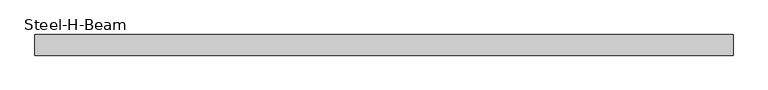
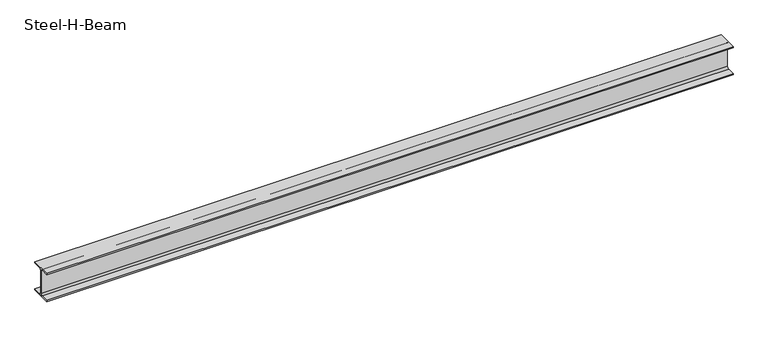
"""IFC4 building model written with IfcOpenShell, lengths in millimetres: beam geometry, Steel-H-Beam : BM121_H-294×200x8x12."""

import ifcopenshell
import ifcopenshell.guid

model = None  # the IFC model being written
_history = None  # IfcOwnerHistory: only IFC2X3 demands one
_inside = {}  # id of a spatial element -> (the spatial element, [elements in it])
_under = {}  # id of a project, library or spatial element -> (it, [spatial elements below it])
_declared = {}  # id of a project -> (the project, [libraries it declares])
_typed = {}  # id of a type object -> (the type object, [elements of that type])
_made_of = {}  # id of a material, layer set ... -> (it, [elements and type objects made of it])


def new_model(schema):
    """Start an empty IFC model of exactly this schema.

    Asked for "IFC4X3", IfcOpenShell would pick the latest addendum, in which some entities
    have other attributes; the version numbers below select the first issue.
    IFC2X3 requires an IfcOwnerHistory on every rooted entity: one is made here for all.
    """
    global model, _history
    if schema == "IFC4X3":
        model = ifcopenshell.file(schema_version=(4, 3, 0, 0))
    else:
        model = ifcopenshell.file(schema=schema)
    _inside.clear()
    _under.clear()
    _declared.clear()
    _typed.clear()
    _made_of.clear()
    _history = None
    if model.schema == "IFC2X3":
        org = make("IfcOrganization", Name="unknown")
        user = make(
            "IfcPersonAndOrganization",
            ThePerson=make("IfcPerson", FamilyName="unknown"),
            TheOrganization=org,
        )
        app = make(
            "IfcApplication",
            ApplicationDeveloper=org,
            Version="unknown",
            ApplicationFullName="unknown",
            ApplicationIdentifier="unknown",
        )
        _history = make(
            "IfcOwnerHistory",
            OwningUser=user,
            OwningApplication=app,
            ChangeAction="ADDED",
            CreationDate=0,
        )
    return model


def make(cls, **values):
    """One entity of the class cls with the attributes given. An attribute that is None is left unset."""
    return model.create_entity(
        cls, **{name: value for name, value in values.items() if value is not None}
    )


def rooted(cls, **values):
    """An entity with a GlobalId (a new one), such as an element, a storey or a relation."""
    return make(cls, GlobalId=ifcopenshell.guid.new(), OwnerHistory=_history, **values)


def si_unit(unit_type, name, prefix=None):
    """IfcSIUnit, for example si_unit("LENGTHUNIT", "METRE", prefix="MILLI")."""
    return make("IfcSIUnit", UnitType=unit_type, Prefix=prefix, Name=name)


def assignment(units):
    """IfcUnitAssignment: the units of a project."""
    return None if units is None else make("IfcUnitAssignment", Units=units)


def point(xyz):
    """IfcCartesianPoint."""
    return None if xyz is None else make("IfcCartesianPoint", Coordinates=xyz)


def direction(xyz):
    """IfcDirection."""
    return None if xyz is None else make("IfcDirection", DirectionRatios=xyz)


def frame(location, z_axis=None, x_axis=None):
    """IfcAxis2Placement3D, a coordinate frame: its origin and axes. An axis left out is left unset."""
    return make(
        "IfcAxis2Placement3D",
        Location=point(location),
        Axis=direction(z_axis),
        RefDirection=direction(x_axis),
    )


def frame_2d(location, x_axis=None):
    """IfcAxis2Placement2D, a coordinate frame in the plane: its origin and x axis."""
    return make(
        "IfcAxis2Placement2D", Location=point(location), RefDirection=direction(x_axis)
    )


def origin():
    """The frame at (0, 0, 0) with its axes left unset."""
    return frame((0.0, 0.0, 0.0))


def place(relative_to, where):
    """IfcLocalPlacement: puts the frame where relative to a parent placement (None: the world)."""
    return make(
        "IfcLocalPlacement", PlacementRelTo=relative_to, RelativePlacement=where
    )


def context(
    kind, dimensions, precision=None, world=None, true_north=None, identifier=None
):
    """IfcGeometricRepresentationContext, for example the 3D "Model" context."""
    return make(
        "IfcGeometricRepresentationContext",
        ContextIdentifier=identifier,
        ContextType=kind,
        CoordinateSpaceDimension=dimensions,
        Precision=precision,
        WorldCoordinateSystem=world,
        TrueNorth=true_north,
    )


def project(units=None, contexts=None):
    """IfcProject with its units and contexts."""
    return rooted(
        "IfcProject",
        Name="project",
        RepresentationContexts=contexts,
        UnitsInContext=assignment(units),
    )


def spatial(cls, under=None, at=None, **own):
    """A site, building, storey or space (cls), placed at a placement, below another one or the project."""
    s = rooted(cls, ObjectPlacement=at, **own)
    if under is not None:
        _under.setdefault(under.id(), (under, []))[1].append(s)
    return s


def polyline(points):
    """IfcPolyline through the points."""
    return make("IfcPolyline", Points=[point(p) for p in points])


def circle_curve(where, radius):
    """IfcCircle in the frame where."""
    return make("IfcCircle", Position=where, Radius=radius)


def trimmed(basis, trim1, trim2, sense, master):
    """IfcTrimmedCurve: the piece of a basis curve between two trims."""
    return make(
        "IfcTrimmedCurve",
        BasisCurve=basis,
        Trim1=trim1,
        Trim2=trim2,
        SenseAgreement=sense,
        MasterRepresentation=master,
    )


def segment(curve, same_sense, transition):
    """IfcCompositeCurveSegment."""
    return make(
        "IfcCompositeCurveSegment",
        Transition=transition,
        SameSense=same_sense,
        ParentCurve=curve,
    )


def composite_curve(segments, self_intersect=None):
    """IfcCompositeCurve: segments joined end to end."""
    return make("IfcCompositeCurve", Segments=segments, SelfIntersect=self_intersect)


def outline(outer, holes=None, kind="AREA"):
    """IfcArbitraryClosedProfileDef: a profile drawn as a closed curve; with holes, ...WithVoids."""
    if holes is None:
        return make("IfcArbitraryClosedProfileDef", ProfileType=kind, OuterCurve=outer)
    return make(
        "IfcArbitraryProfileDefWithVoids",
        ProfileType=kind,
        OuterCurve=outer,
        InnerCurves=holes,
    )


def extrude(swept, where, along, depth):
    """IfcExtrudedAreaSolid: the profile swept, set in the frame where, extruded along a direction by depth."""
    return make(
        "IfcExtrudedAreaSolid",
        SweptArea=swept,
        Position=where,
        ExtrudedDirection=direction(along),
        Depth=depth,
    )


def shape(context_of_items, identifier, shape_type, items):
    """IfcShapeRepresentation: the items that make up one representation, for example the "Body"."""
    return make(
        "IfcShapeRepresentation",
        ContextOfItems=context_of_items,
        RepresentationIdentifier=identifier,
        RepresentationType=shape_type,
        Items=items,
    )


def source(mapping_origin, context_of_items, identifier, shape_type, items):
    """IfcRepresentationMap: a shape defined once, which mapped items show again and again."""
    return make(
        "IfcRepresentationMap",
        MappingOrigin=mapping_origin,
        MappedRepresentation=shape(context_of_items, identifier, shape_type, items),
    )


def transform(
    local_origin,
    x_axis=None,
    y_axis=None,
    z_axis=None,
    scale=None,
    scale2=None,
    scale3=None,
    uniform=True,
):
    """IfcCartesianTransformationOperator3D, or its non-uniform kind. x_axis, y_axis, z_axis: its Axis1, 2, 3."""
    if uniform:
        return make(
            "IfcCartesianTransformationOperator3D",
            Axis1=direction(x_axis),
            Axis2=direction(y_axis),
            LocalOrigin=point(local_origin),
            Scale=scale,
            Axis3=direction(z_axis),
        )
    return make(
        "IfcCartesianTransformationOperator3DnonUniform",
        Axis1=direction(x_axis),
        Axis2=direction(y_axis),
        LocalOrigin=point(local_origin),
        Scale=scale,
        Axis3=direction(z_axis),
        Scale2=scale2,
        Scale3=scale3,
    )


def mapped(mapping_source, mapping_target):
    """IfcMappedItem: shows the shape of a source again, moved by a transform."""
    return make(
        "IfcMappedItem", MappingSource=mapping_source, MappingTarget=mapping_target
    )


def made_of(thing, what):
    """Note that an element or type object is made of a material, layer set ...; save() writes the relation."""
    if what is not None:
        _made_of.setdefault(what.id(), (what, []))[1].append(thing)
    return thing


def element(
    cls,
    number,
    at=None,
    inside=None,
    cuts=None,
    type_object=None,
    material=None,
    context=None,
    identifier="Body",
    shape_type=None,
    held_by="IfcProductDefinitionShape",
    body=None,
    shapes=None,
    **own,
):
    """One element of the class cls, such as IfcWall. Its Tag is "e" and its number.

    at: its placement. inside: the storey or other place that contains it. cuts: it is an
    opening in that element (IfcRelVoidsElement). A single representation is given by context,
    identifier, shape_type and body (its items); several are given by shapes. held_by: the class
    of the entity that holds the representations. save() writes the other relations.
    """
    e = rooted(cls, Tag="e%d" % number, ObjectPlacement=at, **own)
    if body is not None:
        shapes = [shape(context, identifier, shape_type, body)]
    if shapes is not None:
        e.Representation = make(held_by, Representations=shapes)
    if inside is not None:
        _inside.setdefault(inside.id(), (inside, []))[1].append(e)
    if cuts is not None:
        rooted(
            "IfcRelVoidsElement", RelatingBuildingElement=cuts, RelatedOpeningElement=e
        )
    if type_object is not None:
        _typed.setdefault(type_object.id(), (type_object, []))[1].append(e)
    return made_of(e, material)


def aggregate(whole, parts):
    """IfcRelAggregates: a whole, such as a stair, and the parts it consists of."""
    return rooted("IfcRelAggregates", RelatingObject=whole, RelatedObjects=parts)


def save(model, path):
    """Write the relations noted so far, then the file.

    IfcRelAggregates (storeys below a building ...), IfcRelContainedInSpatialStructure (elements
    in a storey), IfcRelDefinesByType, IfcRelAssociatesMaterial and IfcRelDeclares: one each for
    every whole, place, type object, material and project.
    """
    for whole, parts in _under.values():
        aggregate(whole, parts)
    for where, things in _inside.values():
        rooted(
            "IfcRelContainedInSpatialStructure",
            RelatedElements=things,
            RelatingStructure=where,
        )
    for kind, things in _typed.values():
        rooted("IfcRelDefinesByType", RelatedObjects=things, RelatingType=kind)
    for what, things in _made_of.values():
        rooted("IfcRelAssociatesMaterial", RelatedObjects=things, RelatingMaterial=what)
    for by, libraries in _declared.values():
        rooted("IfcRelDeclares", RelatingContext=by, RelatedDefinitions=libraries)
    model.write(path)


def steel_h_beam_013c60b8(model_context):
    return source(origin(), model_context, "Body", "SweptSolid", [
        extrude(outline(composite_curve([segment(polyline([(100.0, -135.0), (100.0, -147.0), (-100.0, -147.0), (-100.0, -135.0), (-22.0, -135.0)]), True, "CONTINUOUS"), segment(trimmed(circle_curve(frame_2d((-22.0, -117.0)), 18.0), [point((-22.0, -135.0))], [point((-4.0, -117.0))], True, "CARTESIAN"), True, "CONTINUOUS"), segment(polyline([(-4.0, -117.0), (-4.0, 117.0)]), True, "CONTINUOUS"), segment(trimmed(circle_curve(frame_2d((-22.0, 117.0)), 18.0), [point((-4.0, 117.0))], [point((-22.0, 135.0))], True, "CARTESIAN"), True, "CONTINUOUS"), segment(polyline([(-22.0, 135.0), (-100.0, 135.0), (-100.0, 147.0), (100.0, 147.0), (100.0, 135.0), (22.0, 135.0)]), True, "CONTINUOUS"), segment(trimmed(circle_curve(frame_2d((22.0, 117.0)), 18.0), [point((22.0, 135.0))], [point((4.0, 117.0))], True, "CARTESIAN"), True, "CONTINUOUS"), segment(polyline([(4.0, 117.0), (4.0, -117.0)]), True, "CONTINUOUS"), segment(trimmed(circle_curve(frame_2d((22.0, -117.0)), 18.0), [point((4.0, -117.0))], [point((22.0, -135.0))], True, "CARTESIAN"), True, "CONTINUOUS"), segment(polyline([(22.0, -135.0), (100.0, -135.0)]), True, "CONTINUOUS")], self_intersect=False)), frame((-3380.0, 0.0, 0.0), z_axis=(1.0, 0.0, 0.0), x_axis=(0.0, 1.0, 0.0)), (0.0, 0.0, 1.0), 6760.0),
    ])


if __name__ == "__main__":
    model = new_model("IFC4")
    model_context = context("Model", 3, world=origin())
    ifc_project = project(units=[si_unit("LENGTHUNIT", "METRE", prefix="MILLI")], contexts=[model_context])
    site = spatial("IfcSite", under=ifc_project)
    building = spatial("IfcBuilding", under=site)
    placement = place(None, origin())
    steel_h_beam_shape = steel_h_beam_013c60b8(model_context)
    element("IfcBeam", 1, ObjectType="Steel-H-Beam : BM121_H-294×200x8x12", at=placement, inside=building, context=model_context, shape_type="MappedRepresentation", body=[
        mapped(steel_h_beam_shape, transform((0.0, 0.0, 0.0), x_axis=(1.0, 0.0, 0.0), y_axis=(0.0, 1.0, 0.0), z_axis=(0.0, 0.0, 1.0))),
    ])
    save(model, "model.ifc")

# Revit data of these elements
# Project information
#   Project ISM Data = "<?xml version=\"1.0\" encoding=\"utf-16\"?><ism schema_version=\"03.00\"><section_positioning><element family_name=\"CO_RC_REC\" symbol_name=\"CCC12_Rec_450x450\" section_id=\"F2ADF140-E21A-4820-8170-6F63D956DCAD\" category=\"OST_StructuralColumns\" mirror_y=\"0\" mirror_x=\"0\" /><element family_name=\"CO_RC_REC\" symbol_name=\"CCC12_Rec_450x450\" section_id=\"B35A310E-4F33-462b-819C-3ADD300C0CEB\" category=\"OST_StructuralColumns\" mirror_y=\"0\" mirror_x=\"0\" /><element family_name=\"CO_RC_REC\" symbol_name=\"CCC12_Rec_450x450\" section_id=\"711054EC-0DB2-46e3-AD20-004560300C00\" category=\"OST_StructuralColumns\" mirror_y=\"0\" mirror_x=\"0\" /><element family_name=\"CO_RC_REC\" symbol_name=\"300 x 450\" section_id=\"B5C54EC9-8EBD-4860-AB72-EF5791AED394\" category=\"OST_StructuralColumns\" mirror_y=\"0\" mirror_x=\"0\" /><element family_name=\"GI_RC_C\" symbol_name=\"SGC11_400x500\" section_id=\"0A7B8D02-9EA4-4aa9-A41A-E30BB5B6B6C5\" category=\"OST_StructuralFraming\" mirror_y=\"0\" mirror_x=\"0\" /><element family_name=\"GI_RC_C\" symbol_name=\"SGC11_400x500\" section_id=\"714BBD27-DB58-47da-B54C-5806291C2D3C\" category=\"OST_StructuralFraming\" mirror_y=\"0\" mirror_x=\"0\" /><element family_name=\"GI_RC_C\" symbol_name=\"SGC11_400x500\" section_id=\"F36E62C1-13EE-4807-A3C1-899E23E0BEDE\" category=\"OST_StructuralFraming\" mirror_y=\"0\" mirror_x=\"0\" /><element family_name=\"GI_RC_C\" symbol_name=\"SGC11_400x500\" section_id=\"F5448801-679E-44d6-8F46-E676344F8165\" category=\"OST_StructuralFraming\" mirror_y=\"0\" mirror_x=\"0\" /><element family_name=\"GI_RC_C\" symbol_name=\"SGC11_400x600\" section_id=\"05D74241-6318-4cac-95F5-7B878260D5B5\" category=\"OST_StructuralFraming\" mirror_y=\"0\" mirror_x=\"0\" /><element family_name=\"GI_RC_C\" symbol_name=\"SGC11_400x500\" section_id=\"846DCB0C-E06B-4978-9D43-E1CC0FDE7595\" category=\"OST_StructuralFraming\" mirror_y=\"0\" mirror_x=\"0\" /><element family_name=\"GI_RC_C\" symbol_name=\"SGC11_400x500\" section_id=\"2ADF82B8-986D-4f44-85DE-89D921292160\" category=\"OST_StructuralFraming\" mirror_y=\"0\" mirror_x=\"0\" /><element family_name=\"GI_RC_C\" symbol_name=\"SGC11_400x500\" section_id=\"7AF371ED-051B-4a30-8826-11F11C212B73\" category=\"OST_StructuralFraming\" mirror_y=\"0\" mirror_x=\"0\" /><element family_name=\"GI_RC_C\" symbol_name=\"SGC11_400x500\" section_id=\"2FE74006-ADDA-412f-A522-853919E62B4D\" category=\"OST_StructuralFraming\" mirror_y=\"0\" mirror_x=\"0\" /><element family_name=\"GI_RC_C\" symbol_name=\"SGC11_400x500\" section_id=\"09B63641-D581-4a6c-A18E-54C17EC989A4\" category=\"OST_StructuralFraming\" mirror_y=\"0\" mirror_x=\"0\" /><element family_name=\"GI_RC_C\" symbol_name=\"SGC11_400x500\" section_id=\"0DD6B52A-77D0-45a1-82B1-8236ED57078C\" category=\"OST_StructuralFraming\" mirror_y=\"0\" mirror_x=\"0\" /><element family_name=\"GI_RC_C\" symbol_name=\"SGC11_400x500\" section_id=\"35D311D2-DEB8-4469-97DE-110B6DF5B84D\" category=\"OST_StructuralFraming\" mirror_y=\"0\" mirror_x=\"0\" /><element family_name=\"GI_RC_C\" symbol_name=\"SGC11_400x500\" section_id=\"0D3CCDE5-CFF9-431b-A4BD-01BF6636D6BD\" category=\"OST_StructuralFraming\" mirror_y=\"0\" mirror_x=\"0\" /><element family_name=\"GI_RC_C\" symbol_name=\"SGC11_400x500\" section_id=\"C62B2A5B-024A-47ac-B030-C17A67E64A7B\" category=\"OST_StructuralFraming\" mirror_y=\"0\" mirror_x=\"0\" /><element family_name=\"GI_RC_C\" symbol_name=\"SGC11_400x500\" section_id=\"944C6E43-E607-48c3-8358-9E6CB88346E7\" category=\"OST_StructuralFraming\" mirror_y=\"0\" mirror_x=\"0\" /><element family_name=\"GI_RC_C\" symbol_name=\"SGC11_400x500\" section_id=\"A4B1F42D-B1C2-4ad2-8AD6-DB0D5E05998D\" category=\"OST_StructuralFraming\" mirror_y=\"0\" mirror_x=\"0\" /><element family_name=\"GI_RC_C\" symbol_name=\"SGC11_400x500\" section_id=\"007E6C70-1139-4b48-B003-C76FAD4C249A\" category=\"OST_StructuralFraming\" mirror_y=\"0\" mirror_x=\"0\" /><element family_name=\"GI_RC_C\" symbol_name=\"SGC11_400x500\" section_id=\"9941AC94-F03A-464c-9912-04590E0C31E0\" category=\"OST_StructuralFraming\" mirror_y=\"0\" mirror_x=\"0\" /><element family_name=\"GI_RC_C\" symbol_name=\"SGC11_400x500\" section_id=\"CFD98B8D-8FF4-4e71-A909-0FE7DBCE924E\" category=\"OST_StructuralFraming\" mirror_y=\"0\" mirror_x=\"0\" /><element family_name=\"GI_RC_C\" symbol_name=\"SGC11_400x500\" section_id=\"58262161-98E6-45c8-B2BD-4508105FF662\" category=\"OST_StructuralFraming\" mirror_y=\"0\" mirror_x=\"0\" /><element family_name=\"GI_RC_C\" symbol_name=\"SGC11_400x500\" section_id=\"66AB4841-610A-4883-97F7-1282A56484E1\" category=\"OST_StructuralFraming\" mirror_y=\"0\" mirror_x=\"0\" /><element family_name=\"GI_RC_C\" symbol_name=\"SGC11_400x500\" section_id=\"D2B324BE-BBD6-49da-9730-60EA7AD4D3A0\" category=\"OST_StructuralFraming\" mirror_y=\"0\" mirror_x=\"0\" /><element family_name=\"GI_RC_C\" symbol_name=\"SGC11_400x500\" section_id=\"92A8ECE7-C053-46b1-92ED-F2C041617E7B\" category=\"OST_StructuralFraming\" mirror_y=\"0\" mirror_x=\"0\" /><element family_name=\"GI_RC_C\" symbol_name=\"SGC11_400x500\" section_id=\"B4C4BDB0-65C4-4016-9C78-DBD77E229523\" category=\"OST_StructuralFraming\" mirror_y=\"0\" mirror_x=\"0\" /><element family_name=\"GI_RC_C\" symbol_name=\"SGC11_400x500\" section_id=\"57270646-162F-4c83-BDB7-A5FBEA9120BD\" category=\"OST_StructuralFraming\" mirror_y=\"0\" mirror_x=\"0\" /><element family_name=\"GI_RC_C\" symbol_name=\"SGC11_400x500\" section_id=\"BDEF733F-00AA-4eee-B6C6-50229FC1D236\" category=\"OST_StructuralFraming\" mirror_y=\"0\" mirror_x=\"0\" /><element family_name=\"GI_RC_C\" symbol_name=\"SGC11_400x500\" section_id=\"84A94E1E-3074-40f4-9690-97191755F019\" category=\"OST_StructuralFraming\" mirror_y=\"0\" mirror_x=\"0\" /><element family_name=\"GI_RC_C\" symbol_name=\"SGC11_400x500\" section_id=\"8A7D913D-7967-4718-912D-B83DF0AD2EDD\" category=\"OST_StructuralFraming\" mirror_y=\"0\" mirror_x=\"0\" /><element family_name=\"GI_RC_C\" symbol_name=\"SGC11_400x500\" section_id=\"83553D70-90FA-469c-B5C3-EF03F3FC6475\" category=\"OST_StructuralFraming\" mirror_y=\"0\" mirror_x=\"0\" /><element family_name=\"GI_RC_C\" symbol_name=\"SGC11_400x500\" section_id=\"6880C1E4-C50B-4c1b-B61C-23F2D8C46873\" category=\"OST_StructuralFraming\" mirror_y=\"0\" mirror_x=\"0\" /><element family_name=\"GI_RC_C\" symbol_name=\"SGC11_400x500\" section_id=\"08594C43-CD40-47de-A3BA-8BFB47F64994\" category=\"OST_StructuralFraming\" mirror_y=\"0\" mirror_x=\"0\" /><element family_name=\"GI_RC_C\" symbol_name=\"SGC11_400x500\" section_id=\"7D2E11FA-A5E1-4434-B9BE-AABA1A16CA03\" category=\"OST_StructuralFraming\" mirror_y=\"0\" mirror_x=\"0\" /><element family_name=\"GI_RC_C\" symbol_name=\"SGC11_400x500\" section_id=\"D892DFA4-5441-4ad2-A390-253492293B1B\" category=\"OST_StructuralFraming\" mirror_y=\"0\" mirror_x=\"0\" /><element family_name=\"GI_RC_C\" symbol_name=\"SGC11_400x500\" section_id=\"E5A32FE6-89C4-49f1-B3B9-1CABE7C48A4D\" category=\"OST_StructuralFraming\" mirror_y=\"0\" mirror_x=\"0\" /><element family_name=\"GI_RC_C\" symbol_name=\"SGC11_400x500\" section_id=\"8AE872C2-5DBE-47c5-934B-7E964A84B589\" category=\"OST_StructuralFraming\" mirror_y=\"0\" mirror_x=\"0\" /><element family_name=\"GI_RC_C\" symbol_name=\"SGC11_400x500\" section_id=\"3C847B60-488A-4604-A400-16A3A65E919B\" category=\"OST_StructuralFraming\" mirror_y=\"0\" mirror_x=\"0\" /><element family_name=\"GI_RC_C\" symbol_name=\"SGC11_400x500\" section_id=\"DBEC432A-3F7B-4266-AD99-2A937DC70BCF\" category=\"OST_StructuralFraming\" mirror_y=\"0\" mirror_x=\"0\" /><element family_name=\"GI_RC_C\" symbol_name=\"SGC11_400x500\" section_id=\"59403DD6-7A51-48aa-A3BE-962457E6F10E\" category=\"OST_StructuralFraming\" mirror_y=\"0\" mirror_x=\"0\" /><element family_name=\"GI_RC_C\" symbol_name=\"SGC11_400x500\" section_id=\"11CDDF5D-38B6-43b2-A291-FC188BE232BC\" category=\"OST_StructuralFraming\" mirror_y=\"0\" mirror_x=\"0\" /><element family_name=\"GI_RC_C\" symbol_name=\"SGC11_400x500\" section_id=\"10BF2843-EFC9-4136-933C-5B270D970277\" category=\"OST_StructuralFraming\" mirror_y=\"0\" mirror_x=\"0\" /><element family_name=\"GI_RC_C\" symbol_name=\"SGC11_400x500\" section_id=\"E1B09A9C-F6C6-47d9-976B-E313C0E3F52B\" category=\"OST_StructuralFraming\" mirror_y=\"0\" mirror_x=\"0\" /><element family_name=\"GI_RC_C\" symbol_name=\"SGC11_400x500\" section_id=\"A3A22EC3-26C8-4588-A0AB-AFAE02DF267E\" category=\"OST_StructuralFraming\" mirror_y=\"0\" mirror_x=\"0\" /><element family_name=\"GI_RC_C\" symbol_name=\"SGC11_400x500\" section_id=\"114828FC-BDC1-4343-9119-BCB5395DAA64\" category=\"OST_StructuralFraming\" mirror_y=\"0\" mirror_x=\"0\" /><element family_name=\"GI_RC_C\" symbol_name=\"SGC11_400x500\" section_id=\"797626F9-3558-4623-826F-15FB93088CB3\" category=\"OST_StructuralFraming\" mirror_y=\"0\" mirror_x=\"0\" /><element family_name=\"GI_RC_C\" symbol_name=\"SGC11_400x500\" section_id=\"4BF369CD-DF09-4346-96CB-C6C6380A2599\" category=\"OST_StructuralFraming\" mirror_y=\"0\" mirror_x=\"0\" /><element family_name=\"GI_RC_C\" symbol_name=\"SGC11_400x500\" section_id=\"722B46BA-61C4-44a1-9ECF-325B60B6688D\" category=\"OST_StructuralFraming\" mirror_y=\"0\" mirror_x=\"0\" /><element family_name=\"GI_RC_C\" symbol_name=\"SGC11_400x500\" section_id=\"C33DBE84-19C1-4379-AB6E-A41F7420F18C\" category=\"OST_StructuralFraming\" mirror_y=\"0\" mirror_x=\"0\" /><element family_name=\"GI_RC_C\" symbol_name=\"SGC11_400x500\" section_id=\"1F2D3B75-66F2-4d88-A1DD-647969477B86\" category=\"OST_StructuralFraming\" mirror_y=\"0\" mirror_x=\"0\" /><element family_name=\"GI_RC_C\" symbol_name=\"SGC11_400x500\" section_id=\"DFBF96B2-410A-4f39-80C4-D8CF78561C93\" category=\"OST_StructuralFraming\" mirror_y=\"0\" mirror_x=\"0\" /><element family_name=\"GI_RC_C\" symbol_name=\"SGC11_400x500\" section_id=\"D6793CD3-AB64-417c-9C28-8B18A0A2D336\" category=\"OST_StructuralFraming\" mirror_y=\"0\" mirror_x=\"0\" /><element family_name=\"GI_RC_C\" symbol_name=\"SGC11_400x500\" section_id=\"90884AC0-EA00-4caa-86E1-E6B886FD90ED\" category=\"OST_StructuralFraming\" mirror_y=\"0\" mirror_x=\"0\" /><element family_name=\"GI_RC_C\" symbol_name=\"SGC11_400x500\" section_id=\"64BC7B89-F7C8-4dae-A5C8-F10DF9E5F6BA\" category=\"OST_StructuralFraming\" mirror_y=\"0\" mirror_x=\"0\" /><element family_name=\"GI_RC_C\" symbol_name=\"SGC11_400x500\" section_id=\"D82E4D85-2728-40e5-9F60-1C7FB2990D78\" category=\"OST_StructuralFraming\" mirror_y=\"0\" mirror_x=\"0\" /><element family_name=\"GI_RC_C\" symbol_name=\"SGC11_400x500\" section_id=\"1E6D05B9-BF84-4669-AA27-948ADA1D511E\" category=\"OST_StructuralFraming\" mirror_y=\"0\" mirror_x=\"0\" /><element family_name=\"GI_RC_C\" symbol_name=\"SGC11_400x500\" section_id=\"73608CB2-EB94-466e-883D-814030EF49D6\" category=\"OST_StructuralFraming\" mirror_y=\"0\" mirror_x=\"0\" /><element family_name=\"GI_RC_C\" symbol_name=\"SGC11_400x500\" section_id=\"4EAF07EF-4E08-4065-9F08-BF69D4413867\" category=\"OST_StructuralFraming\" mirror_y=\"1\" mirror_x=\"1\" /></section_positioning><surface_member_mappings /><element_binding><element revit_id=\"0aa8b22b-49cd-4eb2-b994-d423f7aad482-0014435e\" ism_id=\"637A3C89-B4B9-4EE4-9E04-FF73E7A5771D\" /><element revit_id=\"af7cfdda-f71a-4a09-bb03-63e0c16d5d93-00152efa\" ism_id=\"088C1743-AFAE-4D55-B14F-2330F3A79060\" /><element revit_id=\"af7cfdda-f71a-4a09-bb03-63e0c16d5d93-00152efc\" ism_id=\"38278b30-864a-4bde-bfee-6c2d4309b281\" /><element revit_id=\"af7cfdda-f71a-4a09-bb03-63e0c16d5d93-00152eff\" ism_id=\"e2895b00-887b-4cf1-92a9-c4855f67b579\" /><element revit_id=\"af7cfdda-f71a-4a09-bb03-63e0c16d5d93-00152f02\" ism_id=\"a6b13b86-1938-47ee-8937-754844bb71d9\" /><element revit_id=\"af7cfdda-f71a-4a09-bb03-63e0c16d5d93-00152f05\" ism_id=\"b3cdb4ae-01be-49a8-8521-dfb37fcb7a09\" /><element revit_id=\"af7cfdda-f71a-4a09-bb03-63e0c16d5d93-00152f08\" ism_id=\"0a200294-2d0f-43b2-a10b-c345be42008c\" /><element revit_id=\"af7cfdda-f71a-4a09-bb03-63e0c16d5d
#     93-00152f0a\" ism_id=\"434ac00d-0b75-408a-b526-bf8655b26baf\" /><element revit_id=\"af7cfdda-f71a-4a09-bb03-63e0c16d5d93-00152f0c\" ism_id=\"5e4f7e2a-2154-47cc-93bc-24e7bd197632\" /><element revit_id=\"af7cfdda-f71a-4a09-bb03-63e0c16d5d93-00152f0e\" ism_id=\"f1998cd9-044c-4f7a-99e6-248bc5b45dba\" /><element revit_id=\"af7cfdda-f71a-4a09-bb03-63e0c16d5d93-00152f10\" ism_id=\"6ca0e144-6dd7-4824-b6a4-c3599ffcc64c\" /><element revit_id=\"af7cfdda-f71a-4a09-bb03-63e0c16d5d93-00152f12\" ism_id=\"173f1f07-ca52-4750-b7f6-1ef0180c36ba\" /><element revit_id=\"af7cfdda-f71a-4a09-bb03-63e0c16d5d93-00152f15\" ism_id=\"29a619d1-86ac-46c7-a220-2e78769b313e\" /><element revit_id=\"af7cfdda-f71a-4a09-bb03-63e0c16d5d93-00152f17\" ism_id=\"de21b25d-6b5e-4da6-89ee-8b671f1287ec\" /><element revit_id=\"af7cfdda-f71a-4a09-bb03-63e0c16d5d93-00152f19\" ism_id=\"70cdf538-eeaa-48c4-9315-181e56578638\" /><element revit_id=\"af7cfdda-f71a-4a09-bb03-63e0c16d5d93-00152f1b\" ism_id=\"49734cf8-a963-4163-b104-a25bff74fff0\" /><element revit_id=\"af7cfdda-f71a-4a09-bb03-63e0c16d5d93-00152f1d\" ism_id=\"a5a98e28-e98d-4759-bcab-d40632bfc19f\" /><element revit_id=\"af7cfdda-f71a-4a09-bb03-63e0c16d5d93-00152f1f\" ism_id=\"ab6af08f-90da-4d2f-a66a-db65621b8e94\" /><element revit_id=\"af7cfdda-f71a-4a09-bb03-63e0c16d5d93-00152f21\" ism_id=\"a65b64ab-134d-4223-82b7-5e66d90bc276\" /><element revit_id=\"af7cfdda-f71a-4a09-bb03-63e0c16d5d93-00152f23\" ism_id=\"6a1f317f-8940-4af8-9522-8e6c47c0c3a6\" /><element revit_id=\"af7cfdda-f71a-4a09-bb03-63e0c16d5d93-00152f25\" ism_id=\"880c6aab-7058-4382-9d83-6c759bdcf822\" /><element revit_id=\"af7cfdda-f71a-4a09-bb03-63e0c16d5d93-00152f27\" ism_id=\"555977b1-6494-4ee8-b235-8bae97762787\" /><element revit_id=\"af7cfdda-f71a-4a09-bb03-63e0c16d5d93-00152f29\" ism_id=\"66c9b467-8c65-4f1e-9542-95b43d793e9b\" /><element revit_id=\"af7cfdda-f71a-4a09-bb03-63e0c16d5d93-00152f2b\" ism_id=\"217a9ce2-64ab-4115-836e-06014fa1b21e\" /><element revit_id=\"af7cfdda-f71a-4a09-bb03-63e0c16d5d93-00152f2d\" ism_id=\"f7fc30da-832d-44e7-bab3-dd115d25639e\" /><element revit_id=\"af7cfdda-f71a-4a09-bb03-63e0c16d5d93-00152f2f\" ism_id=\"715eb46c-1b8d-4226-a7c6-6c6c165bf34d\" /><element revit_id=\"af7cfdda-f71a-4a09-bb03-63e0c16d5d93-00152f31\" ism_id=\"ef53c2b2-6fcf-42d2-96ea-f30a899bf64f\" /><element revit_id=\"af7cfdda-f71a-4a09-bb03-63e0c16d5d93-00152f34\" ism_id=\"1aefa093-18ee-4a97-8178-1b1fb4b7aceb\" /><element revit_id=\"af7cfdda-f71a-4a09-bb03-63e0c16d5d93-00152f38\" ism_id=\"262f02a9-64ca-487b-befd-4b58d44dffa7\" /><element revit_id=\"af7cfdda-f71a-4a09-bb03-63e0c16d5d93-00152f3b\" ism_id=\"6f2442a8-c4c0-4b53-9d7f-7059d6ededd2\" /><element revit_id=\"af7cfdda-f71a-4a09-bb03-63e0c16d5d93-00152f3e\" ism_id=\"dd838df4-69c7-406c-93e1-418c01f5734f\" /><element revit_id=\"af7cfdda-f71a-4a09-bb03-63e0c16d5d93-00152f40\" ism_id=\"9dec5077-28a7-4c32-95d2-08813de6a916\" /><element revit_id=\"af7cfdda-f71a-4a09-bb03-63e0c16d5d93-00152f42\" ism_id=\"9370ae5f-9277-4bb3-917b-cb3f318800a8\" /><element revit_id=\"af7cfdda-f71a-4a09-bb03-63e0c16d5d93-00152f44\" ism_id=\"0f3f2c81-58b4-4698-b1be-75061a4a2ae1\" /><element revit_id=\"af7cfdda-f71a-4a09-bb03-63e0c16d5d93-00152f46\" ism_id=\"95dca10f-6510-4ae7-a23e-7a1fd6939662\" /><element revit_id=\"af7cfdda-f71a-4a09-bb03-63e0c16d5d93-00152f49\" ism_id=\"83bad907-6a1c-4702-9990-a1a9c13d0160\" /><element revit_id=\"af7cfdda-f71a-4a09-bb03-63e0c16d5d93-00152f4d\" ism_id=\"7dba72dc-0de8-457c-8d3c-9c80941133ff\" /><element revit_id=\"af7cfdda-f71a-4a09-bb03-63e0c16d5d93-00152f51\" ism_id=\"a6cf3de2-949b-45b4-8029-061e06e5ab91\" /><element revit_id=\"af7cfdda-f71a-4a09-bb03-63e0c16d5d93-00152f54\" ism_id=\"77af5754-dd62-4c90-accb-d0b9405b5baf\" /><element revit_id=\"af7cfdda-f71a-4a09-bb03-63e0c16d5d93-00152f56\" ism_id=\"6461cb37-823d-49bb-bea2-3dbd4db85a81\" /><element revit_id=\"af7cfdda-f71a-4a09-bb03-63e0c16d5d93-00152f59\" ism_id=\"e2f2909f-27bc-426e-b2db-27b1217d3560\" /><element revit_id=\"af7cfdda-f71a-4a09-bb03-63e0c16d5d93-00152f5b\" ism_id=\"46c410de-fc65-4593-ae24-da1a154b45fb\" /><element revit_id=\"af7cfdda-f71a-4a09-bb03-63e0c16d5d93-00152f5d\" ism_id=\"d7d73cf7-a31f-421c-bc39-3ba338a334b1\" /><element revit_id=\"af7cfdda-f71a-4a09-bb03-63e0c16d5d93-00152f61\" ism_id=\"6bd81f7b-5fd8-4f19-ad3a-4e009274854c\" /><element revit_id=\"af7cfdda-f71a-4a09-bb03-63e0c16d5d93-00152f64\" ism_id=\"f25b9af0-504f-4aaf-a359-d2bc9d32b683\" /><element revit_id=\"af7cfdda-f71a-4a09-bb03-63e0c16d5d93-00152f66\" ism_id=\"f143dcd3-1cc7-47ae-b4ed-c960a7d1349c\" /><element revit_id=\"af7cfdda-f71a-4a09-bb03-63e0c16d5d93-00152f68\" ism_id=\"296e8d7f-a89b-405a-b793-fc1ea4b11be5\" /><element revit_id=\"af7cfdda-f71a-4a09-bb03-63e0c16d5d93-00152f6b\" ism_id=\"48b24488-3184-439c-b285-73e81edfef17\" /><element revit_id=\"af7cfdda-f71a-4a09-bb03-63e0c16d5d93-00152f6e\" ism_id=\"0db0ccd4-631c-4972-aad8-2fd483c55629\" /><element revit_id=\"af7cfdda-f71a-4a09-bb03-63e0c16d5d93-00152f71\" ism_id=\"ee51bd40-01d8-4a48-92c6-90509a96cad2\" /><element revit_id=\"af7cfdda-f71a-4a09-bb03-63e0c16d5d93-00152f73\" ism_id=\"e5c66ce6-ca9d-4591-9d75-5348307a88bc\" /><element revit_id=\"af7cfdda-f71a-4a09-bb03-63e0c16d5d93-00152f75\" ism_id=\"892d82ae-6f73-4af5-8575-78955f2b6c3b\" /><element revit_id=\"af7cfdda-f71a-4a09-bb03-63e0c16d5d93-00152f78\" ism_id=\"cb5b2a2e-5551-4b87-9d0b-6382c09e6ce2\" /><element revit_id=\"af7cfdda-f71a-4a09-bb03-63e0c16d5d93-00152f7c\" ism_id=\"1177c4ab-d04b-426b-80ba-afa1f1403e20\" /><element revit_id=\"af7cfdda-f71a-4a09-bb03-63e0c16d5d93-00152f7f\" ism_id=\"235d8a18-f10a-44ad-8945-ebb2f02646fa\" /><element revit_id=\"af7cfdda-f71a-4a09-bb03-63e0c16d5d93-00152f83\" ism_id=\"6127db9d-7d4b-44c8-806c-e4f7d278db0c\" /><element revit_id=\"af7cfdda-f71a-4a09-bb03-63e0c16d5d93-00152f86\" ism_id=\"85d79da8-d317-4e5b-88a2-88d20cb73d7d\" /><element revit_id=\"af7cfdda-f71a-4a09-bb03-63e0c16d5d93-00152f89\" ism_id=\"f4105a19-7c5e-4970-9446-50e578b67af2\" /><element revit_id=\"af7cfdda-f71a-4a09-bb03-63e0c16d5d93-00152f8b\" ism_id=\"ab299061-87b1-4edc-8a5c-c55542368f39\" /><element revit_id=\"af7cfdda-f71a-4a09-bb03-63e0c16d5d93-00152f8d\" ism_id=\"43097401-25be-48d4-a7ba-f3c37c1b84e9\" /><element revit_id=\"af7cfdda-f71a-4a09-bb03-63e0c16d5d93-00152f8f\" ism_id=\"fd9214b7-59e9-4736-b544-a37d4c180e24\" /><element revit_id=\"af7cfdda-f71a-4a09-bb03-63e0c16d5d93-00152f91\" ism_id=\"b83d1d95-2d97-4532-8a94-368577601c17\" /><element revit_id=\"af7cfdda-f71a-4a09-bb03-63e0c16d5d93-00152f94\" ism_id=\"9bd5e620-e2eb-4ede-9a8b-b0183e171248\" /><element revit_id=\"af7cfdda-f71a-4a09-bb03-63e0c16d5d93-00152f97\" ism_id=\"d6f9d903-1605-43dc-872c-2f9de6642af6\" /><element revit_id=\"af7cfdda-f71a-4a09-bb03-63e0c16d5d93-00152f99\" ism_id=\"7c236b12-3da8-4ae0-bc99-2aa089118476\" /><element revit_id=\"af7cfdda-f71a-4a09-bb03-63e0c16d5d93-00152f9b\" ism_id=\"2b88d03d-aeef-4f51-b98c-562513d6f6da\" /><element revit_id=\"af7cfdda-f71a-4a09-bb03-63e0c16d5d93-00152f9d\" ism_id=\"6639b07f-6759-4580-bc0a-91cdbc82216d\" /><element revit_id=\"af7cfdda-f71a-4a09-bb03-63e0c16d5d93-00152f9f\" ism_id=\"d17e7cf5-d760-4c38-8bb0-8a57fe45e3ad\" /><element revit_id=\"af7cfdda-f71a-4a09-bb03-63e0c16d5d93-00152fa2\" ism_id=\"6dbdf2a2-22ac-4132-a9ae-8992fe15b0d7\" /><element revit_id=\"af7cfdda-f71a-4a09-bb03-63e0c16d5d93-00152fa4\" ism_id=\"663381be-9f3f-499f-b7c1-64170401ecb3\" /><element revit_id=\"af7cfdda-f71a-4a09-bb03-63e0c16d5d93-00152fa6\" ism_id=\"5ba3ff14-3d24-47a8-9418-aecce16bd943\" /><element revit_id=\"af7cfdda-f71a-4a09-bb03-63e0c16d5d93-00152fa8\" ism_id=\"8f845e6a-1432-4c61-8362-e12c105320fb\" /><element revit_id=\"af7cfdda-f71a-4a09-bb03-63e0c16d5d93-00152faa\" ism_id=\"263897bf-02c2-4ed7-8e3f-2020d545125e\" /><element revit_id=\"af7cfdda-f71a-4a09-bb03-63e0c16d5d93-00152fac\" ism_id=\"f1241312-d990-4c87-92ff-afc1975a3d67\" /><element revit_id=\"af7cfdda-f71a-4a09-bb03-63e0c16d5d93-00152fae\" ism_id=\"5740cb23-0cbc-47ce-acea-31b5a043bf0c\" /><element revit_id=\"af7cfdda-f71a-4a09-bb03-63e0c16d5d93-00152fb0\" ism_id=\"7aeaeafb-f9bc-4bee-b237-caade22069b8\" /><element revit_id=\"af7cfdda-f71a-4a09-bb03-63e0c16d5d93-00152fb3\" ism_id=\"90084dda-e197-4e46-8e5b-4f629a594830\" /><element revit_id=\"af7cfdda-f71a-4a09-bb03-63e0c16d5d93-00152fb5\" ism_id=\"2c392f12-2b50-4bd2-8c41-ef64640e587b\" /><element revit_id=\"af7cfdda-f71a-4a09-bb03-63e0c16d5d93-00152fb7\" ism_id=\"d25284c0-6931-4cbb-8ed3-63397f6a5616\" /><element revit_id=\"af7cfdda-f71a-4a09-bb03-63e0c16d5d93-00152fb9\" ism_id=\"32799d39-e9bc-468c-ac64-a3f2c8e075af\" /><element revit_id=\"af7cfdda-f71a-4a09-bb03-63e0c16d5d93-00152fbb\" ism_id=\"61a092b8-d924-4e61-a1ef-adc051541aaf\" /><element revit_id=\"af7cfdda-f71a-4a09-bb03-63e0c16d5d93-00152fbe\" ism_id=\"ae89ad42-0006-42ee-9328-01a896002b7a\" /><element revit_id=\"af7cfdda-f71a-4a09-bb03-63e0c16d5d93-00152fc0\" ism_id=\"7b4d47fd-5fcd-4692-9b39-36bb95372647\" /><element revit_id=\"af7cfdda-f71a-4a09-bb03-63e0c16d5d93-00152fc2\" ism_id=\"150f022d-eb78-47d8-8d70-c7ea5433f366\" /><element revit_id=\"af7cfdda-f71a-4a09-bb03-63e0c16d5d93-00152fc4\" ism_id=\"6780451e-52c6-4962-8bb4-f1fd57bf7865\" /><element revit_id=\"af7cfdda-f71a-4a09-bb03-63e0c16d5d93-00152fc6\" ism_id=\"b3896748-2d7c-424b-ae81-8b769d840fbc\" /><element revit_id=\"af7cfdda-f71a-4a09-bb03-63e0c16d5d93-00152fc9\" ism_id=\"0c64c745-ce95-4f37-8a9d-d07fd5d17ecb\" /><element revit_id=\"af7cfdda-f71a-4a09-bb03-63e0c16d5d93-00152fcc\" ism_id=\"dc23390d-d501-4d7e-9369-f7793a7306a7\" /><element revit_id=\"af7cfdda-f71a-4a09-bb03-63e0c16d5d93-00152fcf\" ism_id=\"a2d2dfc7-08e7-459b-9de9-2d46c1b9d65d\" /><element revit_id=\"af7cfdda-f71a-4a09-bb03-63e0c16d5d93-00152fd2\" ism_id=\"0357c393-c221-46b8-a525-7eece05024d5\" /><element revit_id=\"af7cfdda-f71a-4a09-bb03-63e0c16d5d93-00152fd4\" ism_id=\"7514ec1a-cc54-428f-bbfe-53465c7b9971\" /><element revit_id=\"af7cfdda-f71a-4a09-bb03-63e0c16d5d93-00152fd7\" ism_id=\"f5e61f1a-565d-4eed-b8cc-74798bf49f83\" /><element revit_id=\"af7cfdda-f71a-4a09-bb03-63e0c16d5d93-00152fd9\" ism_id=\"7d7031a0-6061-49e6-8bb3-df1503ddb602\" /><element revit_id=\"af7cfdda-f71a-4a09-bb03-63e0c16d5d93-00152fdb\" ism_id=\"0d733cbc-e2dd-44ec-a5f3-da43d2d7ec46\" /><element revit_id=\"af7cfdda-f71a-4a09-bb03-63e0c16d5d93-00152fdd\" ism_id=\"21cbc8e9-c640-4a2e-8958-1d3b7a784879\" /><element revit_id=\"af7cfdda-f71a-4a09-bb03-63e0c16d5d93-00152fdf\" ism_id=\"fac86bbb-1d81-4320-81cd-30997be31eb4\" /><element revit_id=\"af7cfdda-f71a-4a09-bb03-63e0c16d5d93-00152fe1\" ism_id=\"ebc7c696-170e-4ba4-8599-103279d331b8\" /><element revit_id=\"af7cfdda-f71a-4a09-bb03-63e0c16d5d93-00152fe3\" ism_id=\"91dec439-7fd8-4259-bbce-df46237765e2\" /><element revit_id=\"af7cfdda-f71a-4a09-bb03-63e0c16d5d93-00152fe5\" ism_id=\"6227503a-c521-4b5a-b5c3-b9e2ea2b5c81\" /><element revit_id=\"af7cfdda-f71a-4a09-bb03-63e0c16d5d93-00152fe7\" ism_id=\"e6e91966-53ab-4536-84a0-3f6e5a22fbeb\" /><element revit_id=\"af7cfdda-f71a-4a09-bb03-63e0c16d5d93-00152fe9\" ism_id=\"fb3387b3-301c-40a5-8217-97be67c50843\" /><element revit_id=\"af7cfdda-f71a-4a09-bb03-63e0c16d5d93-00152feb\" ism_id=\"37825fc8-0fe2-440e-933a-1453c922c9d9\" /><element revit_id=\"af7cfdda-f71a-4a09-bb03-63e0c16d5d93-00152fed\" ism_id=\"06b175df-5526-4920-a3d6-7f2ff872756e\" /><element revit_id=\"af7cfdda-f71a-4a09-bb03-63e0c16d5d93-00152fef\" ism_id=\"a8fbce7a-6989-46e5-9bc5-c497d4a295c9\" /><element revit_id=\"af7cfdda-f71a-4a09-bb03-63e0c16d5d93-00152ff1\" ism_id=\"cf8ccf89-d0da-4b4e-93d8-85d639853d5e\" /><element revit_id=\"af7cfdda-f71a-4a09-bb03-63e0c16d5d93-00152ff3\" ism_id=\"1b85e87c-6c2a-4057-8491-40e4237cd0e6\" /><element revit_id=\"af7cfdda-f71a-4a09-bb03-63e0c16d5d93-00152ff5\" ism_id=\"69be497f-343c-4d38-9ea0-e959474332f8\" /><element revit_id=\"af7cfdda-f71a-4a09-bb03-63e0c16d5d93-00152ff7\" ism_id=\"72738956-f87a-41b4-a019-35adc3bff764\" /><element revit_id=\"af7cfdda-f71a-4a09-bb03-63e0c16d5d93-00152ff9\" ism_id=\"f127b15c-142d-4b57-83a6-5b76ac4cde6e\" /><element revit_id=
#     \"af7cfdda-f71a-4a09-bb03-63e0c16d5d93-00152ffb\" ism_id=\"3a38a709-bfa8-404e-b889-5af5e78ea0bf\" /><element revit_id=\"af7cfdda-f71a-4a09-bb03-63e0c16d5d93-00152ffe\" ism_id=\"bebf0363-7e59-4a43-8f5b-502fcc4a338d\" /><element revit_id=\"af7cfdda-f71a-4a09-bb03-63e0c16d5d93-00153000\" ism_id=\"157fe154-0d28-4e8c-a143-e2896867fd28\" /><element revit_id=\"af7cfdda-f71a-4a09-bb03-63e0c16d5d93-00153002\" ism_id=\"1bf52bf8-7327-4d55-b5cd-bf7c9bf89688\" /><element revit_id=\"af7cfdda-f71a-4a09-bb03-63e0c16d5d93-00153005\" ism_id=\"7a0025bf-d54b-4614-9002-7bd4a82da90e\" /><element revit_id=\"af7cfdda-f71a-4a09-bb03-63e0c16d5d93-00153008\" ism_id=\"cad53638-8c8f-4a89-ab6f-d8a32131833b\" /><element revit_id=\"af7cfdda-f71a-4a09-bb03-63e0c16d5d93-0015300a\" ism_id=\"05672ccd-1a96-434c-8da1-7a706b3561f7\" /><element revit_id=\"af7cfdda-f71a-4a09-bb03-63e0c16d5d93-0015300c\" ism_id=\"bb809016-b2bb-4157-847e-1cca3692ba19\" /><element revit_id=\"af7cfdda-f71a-4a09-bb03-63e0c16d5d93-0015300f\" ism_id=\"720ed192-8aa7-46fd-9f7a-15d64351767c\" /><element revit_id=\"af7cfdda-f71a-4a09-bb03-63e0c16d5d93-00153011\" ism_id=\"9a47cdb9-976d-41f3-a5c3-5a7516a7763c\" /><element revit_id=\"af7cfdda-f71a-4a09-bb03-63e0c16d5d93-00153013\" ism_id=\"aba01787-c82b-453e-8db2-70277a34d5ad\" /><element revit_id=\"af7cfdda-f71a-4a09-bb03-63e0c16d5d93-00153015\" ism_id=\"f6b882e3-d64a-44b1-878c-9c00ee1fde86\" /><element revit_id=\"af7cfdda-f71a-4a09-bb03-63e0c16d5d93-00153017\" ism_id=\"95108815-490a-427a-aec1-8fcefc57c858\" /><element revit_id=\"af7cfdda-f71a-4a09-bb03-63e0c16d5d93-00153019\" ism_id=\"8fe55cf1-56b4-4a62-948a-d7f0c95bd04b\" /><element revit_id=\"af7cfdda-f71a-4a09-bb03-63e0c16d5d93-0015301b\" ism_id=\"b889bf8b-3bdd-410a-b11b-9ca69449d470\" /><element revit_id=\"af7cfdda-f71a-4a09-bb03-63e0c16d5d93-0015301d\" ism_id=\"ef8604de-de5b-45ec-9158-0b702e6ef713\" /><element revit_id=\"af7cfdda-f71a-4a09-bb03-63e0c16d5d93-0015301f\" ism_id=\"40ee286a-4bc9-4d4f-ba6d-fe1ac9da03cf\" /><element revit_id=\"af7cfdda-f71a-4a09-bb03-63e0c16d5d93-00153021\" ism_id=\"cc903f39-6bdf-4081-a56c-883169221735\" /><element revit_id=\"af7cfdda-f71a-4a09-bb03-63e0c16d5d93-00153023\" ism_id=\"0af04955-dcb6-4295-b3d4-7c432a233062\" /><element revit_id=\"af7cfdda-f71a-4a09-bb03-63e0c16d5d93-00153025\" ism_id=\"75a51549-6a04-4399-b818-f170a8c10286\" /><element revit_id=\"af7cfdda-f71a-4a09-bb03-63e0c16d5d93-00153027\" ism_id=\"7e183794-5c66-46bc-97f5-2df209b3286d\" /><element revit_id=\"af7cfdda-f71a-4a09-bb03-63e0c16d5d93-00153029\" ism_id=\"ed4a7448-29b0-44e3-8b6f-7310f83440ab\" /><element revit_id=\"af7cfdda-f71a-4a09-bb03-63e0c16d5d93-0015302b\" ism_id=\"fdb5eb17-b94e-40c1-b703-3ecb5e4efee4\" /><element revit_id=\"af7cfdda-f71a-4a09-bb03-63e0c16d5d93-0015302d\" ism_id=\"779397c1-65b7-447f-a72e-2a09308021ea\" /><element revit_id=\"af7cfdda-f71a-4a09-bb03-63e0c16d5d93-0015302f\" ism_id=\"7b409707-86c5-44e2-919e-92ad5bb9eb8b\" /><element revit_id=\"af7cfdda-f71a-4a09-bb03-63e0c16d5d93-00153031\" ism_id=\"d337c78b-590d-406c-bf20-6a3558821db1\" /><element revit_id=\"af7cfdda-f71a-4a09-bb03-63e0c16d5d93-00153033\" ism_id=\"c27f5f6d-8445-4415-853d-d316787bea6e\" /><element revit_id=\"af7cfdda-f71a-4a09-bb03-63e0c16d5d93-00153035\" ism_id=\"76036a55-3bab-417a-ba41-ec1335e2e2a7\" /><element revit_id=\"af7cfdda-f71a-4a09-bb03-63e0c16d5d93-00153037\" ism_id=\"24be638c-ff89-4616-8974-5b79c81e6e56\" /><element revit_id=\"af7cfdda-f71a-4a09-bb03-63e0c16d5d93-00153039\" ism_id=\"015f9f2c-2353-4795-b891-e4ee986f25f7\" /><element revit_id=\"af7cfdda-f71a-4a09-bb03-63e0c16d5d93-0015303b\" ism_id=\"91f8ddfb-c5b9-4f33-b141-a6edfbccf098\" /><element revit_id=\"af7cfdda-f71a-4a09-bb03-63e0c16d5d93-0015303d\" ism_id=\"78540364-1ba5-4f0c-95fb-ba8631e32695\" /><element revit_id=\"af7cfdda-f71a-4a09-bb03-63e0c16d5d93-0015303f\" ism_id=\"9d53e406-367b-4e3e-b5e8-d421731e1aab\" /><element revit_id=\"af7cfdda-f71a-4a09-bb03-63e0c16d5d93-00153041\" ism_id=\"24aa6051-1a20-4f08-8962-6f6f9ff4dc98\" /><element revit_id=\"af7cfdda-f71a-4a09-bb03-63e0c16d5d93-00153043\" ism_id=\"572a4144-5250-4962-a1b9-09502cda2774\" /><element revit_id=\"af7cfdda-f71a-4a09-bb03-63e0c16d5d93-00153045\" ism_id=\"1f486980-0be9-4aad-b32e-0608218bf68e\" /><element revit_id=\"af7cfdda-f71a-4a09-bb03-63e0c16d5d93-00153047\" ism_id=\"588ed856-d113-4521-b97c-a4d7ac7ba406\" /><element revit_id=\"af7cfdda-f71a-4a09-bb03-63e0c16d5d93-00153049\" ism_id=\"741942b7-995d-48cb-8401-4faec8ef8d15\" /><element revit_id=\"af7cfdda-f71a-4a09-bb03-63e0c16d5d93-0015304b\" ism_id=\"85254c30-08c9-46e3-acd6-6b5131f485ce\" /><element revit_id=\"af7cfdda-f71a-4a09-bb03-63e0c16d5d93-0015304e\" ism_id=\"2d57d6c0-67d8-48bd-b16f-8ef7edb485b1\" /><element revit_id=\"af7cfdda-f71a-4a09-bb03-63e0c16d5d93-00153050\" ism_id=\"57b4caff-473e-4ebc-b42c-d73ce4ca67d8\" /><element revit_id=\"af7cfdda-f71a-4a09-bb03-63e0c16d5d93-00153052\" ism_id=\"1adae240-a487-478c-a898-61bee40e7415\" /><element revit_id=\"af7cfdda-f71a-4a09-bb03-63e0c16d5d93-00153054\" ism_id=\"62613b5f-092e-4f63-86ac-d3e070a85bc5\" /><element revit_id=\"af7cfdda-f71a-4a09-bb03-63e0c16d5d93-00153056\" ism_id=\"6aecb1de-b991-4eed-80ad-e1b9ccc03a87\" /><element revit_id=\"af7cfdda-f71a-4a09-bb03-63e0c16d5d93-00153058\" ism_id=\"ecab5d8d-84d0-44a4-9549-bca959ac514b\" /><element revit_id=\"af7cfdda-f71a-4a09-bb03-63e0c16d5d93-0015305a\" ism_id=\"589f44ad-061b-46bc-91bd-bf9b1e708415\" /><element revit_id=\"af7cfdda-f71a-4a09-bb03-63e0c16d5d93-0015305c\" ism_id=\"bfa24af8-499f-45ff-9e9d-d5cc0761fed6\" /><element revit_id=\"af7cfdda-f71a-4a09-bb03-63e0c16d5d93-0015305e\" ism_id=\"8114f473-ca73-4cc8-b3e2-979f07368f66\" /><element revit_id=\"af7cfdda-f71a-4a09-bb03-63e0c16d5d93-00153060\" ism_id=\"4dde7439-2ac9-412f-a5f5-e9fd0f294ec8\" /><element revit_id=\"af7cfdda-f71a-4a09-bb03-63e0c16d5d93-00153062\" ism_id=\"661cc7d8-fd9c-4505-b43e-241bfd24b2d0\" /><element revit_id=\"af7cfdda-f71a-4a09-bb03-63e0c16d5d93-00153064\" ism_id=\"1e7f186f-1b55-4d4c-bf9f-18595049605e\" /><element revit_id=\"af7cfdda-f71a-4a09-bb03-63e0c16d5d93-00153066\" ism_id=\"ee968183-c9c6-4eab-86cf-0eda12de724b\" /><element revit_id=\"af7cfdda-f71a-4a09-bb03-63e0c16d5d93-00153068\" ism_id=\"5de1f319-cdd1-4b9a-8f8e-b86394effa22\" /><element revit_id=\"af7cfdda-f71a-4a09-bb03-63e0c16d5d93-0015306a\" ism_id=\"fa557a6c-2e39-4481-9eb5-5ede8fd31c49\" /><element revit_id=\"af7cfdda-f71a-4a09-bb03-63e0c16d5d93-0015306c\" ism_id=\"b2710e8e-0f5f-4e74-a366-aef04da22cd3\" /><element revit_id=\"af7cfdda-f71a-4a09-bb03-63e0c16d5d93-0015306e\" ism_id=\"5633c3b7-f903-46ee-b126-8a20a9a62c90\" /><element revit_id=\"af7cfdda-f71a-4a09-bb03-63e0c16d5d93-00153070\" ism_id=\"62796ef8-c4bb-4b9f-bd14-cc7392046eb4\" /><element revit_id=\"af7cfdda-f71a-4a09-bb03-63e0c16d5d93-00153072\" ism_id=\"db898ada-150e-4ff5-a9f8-16e27b46b754\" /><element revit_id=\"af7cfdda-f71a-4a09-bb03-63e0c16d5d93-00153075\" ism_id=\"d3965d2d-e119-4f6b-af8d-52c8a5397d36\" /><element revit_id=\"af7cfdda-f71a-4a09-bb03-63e0c16d5d93-00153077\" ism_id=\"063574e4-6319-4ba7-8e34-1638a1357d5f\" /><element revit_id=\"af7cfdda-f71a-4a09-bb03-63e0c16d5d93-00153079\" ism_id=\"6de69805-8980-44f0-9316-6d50d1b47cbb\" /><element revit_id=\"af7cfdda-f71a-4a09-bb03-63e0c16d5d93-0015307b\" ism_id=\"e5f77c5b-4806-4993-8875-6149db708e42\" /><element revit_id=\"af7cfdda-f71a-4a09-bb03-63e0c16d5d93-0015307d\" ism_id=\"a13071c9-c086-4896-95a6-a015bc531f25\" /><element revit_id=\"af7cfdda-f71a-4a09-bb03-63e0c16d5d93-0015307f\" ism_id=\"c9d216f9-adca-4752-b8c1-d779727505dd\" /><element revit_id=\"af7cfdda-f71a-4a09-bb03-63e0c16d5d93-00153081\" ism_id=\"5b167621-3850-4169-8bee-1e0420bf6050\" /><element revit_id=\"af7cfdda-f71a-4a09-bb03-63e0c16d5d93-00153083\" ism_id=\"09cf76ae-a083-4203-a622-7e9424374f66\" /><element revit_id=\"af7cfdda-f71a-4a09-bb03-63e0c16d5d93-00153085\" ism_id=\"14063b50-058d-464a-aa08-369865983eeb\" /><element revit_id=\"af7cfdda-f71a-4a09-bb03-63e0c16d5d93-00153087\" ism_id=\"add5837f-63be-4349-b708-9f4051059e25\" /><element revit_id=\"af7cfdda-f71a-4a09-bb03-63e0c16d5d93-00153089\" ism_id=\"b4c60bd3-61cb-423f-916a-fa2b71585228\" /><element revit_id=\"af7cfdda-f71a-4a09-bb03-63e0c16d5d93-0015308b\" ism_id=\"6251d90e-381f-4771-818c-f7465ae91864\" /><element revit_id=\"af7cfdda-f71a-4a09-bb03-63e0c16d5d93-0015308d\" ism_id=\"7693be9d-48ca-4005-bed4-90e9c08d3a38\" /><element revit_id=\"af7cfdda-f71a-4a09-bb03-63e0c16d5d93-0015308f\" ism_id=\"a6a39ca9-cd56-43ba-bfe8-2cf3b78878cc\" /><element revit_id=\"af7cfdda-f71a-4a09-bb03-63e0c16d5d93-00153091\" ism_id=\"1a3956c4-77bb-4ccc-a12d-c3514cf365d4\" /><element revit_id=\"af7cfdda-f71a-4a09-bb03-63e0c16d5d93-00153093\" ism_id=\"2ffa7a89-8ee9-470a-b3d8-7c27f566e226\" /><element revit_id=\"af7cfdda-f71a-4a09-bb03-63e0c16d5d93-00153095\" ism_id=\"e865b460-944f-4057-a6e8-4e39cb88d97d\" /><element revit_id=\"af7cfdda-f71a-4a09-bb03-63e0c16d5d93-00153097\" ism_id=\"69410bb9-8440-4a88-9151-b5459095fe2e\" /><element revit_id=\"af7cfdda-f71a-4a09-bb03-63e0c16d5d93-00153099\" ism_id=\"1efae87b-0246-432c-a428-82c87fb3929c\" /><element revit_id=\"af7cfdda-f71a-4a09-bb03-63e0c16d5d93-0015309b\" ism_id=\"e1d5fb57-3b5d-4a32-bccb-cea278671f2f\" /><element revit_id=\"af7cfdda-f71a-4a09-bb03-63e0c16d5d93-0015309d\" ism_id=\"c74a7061-f4b2-41b5-b3ff-caf6cf9dfffd\" /><element revit_id=\"af7cfdda-f71a-4a09-bb03-63e0c16d5d93-0015309f\" ism_id=\"aa777ec3-1257-49eb-b597-fbab7bda8b11\" /><element revit_id=\"af7cfdda-f71a-4a09-bb03-63e0c16d5d93-001530a1\" ism_id=\"7420a67b-bb48-477d-823a-c473ce92c083\" /><element revit_id=\"af7cfdda-f71a-4a09-bb03-63e0c16d5d93-001530a3\" ism_id=\"1ee9340a-8778-4cd6-be2d-57fb5fe16e45\" /><element revit_id=\"af7cfdda-f71a-4a09-bb03-63e0c16d5d93-001530a5\" ism_id=\"3216ac21-29b0-45a7-a070-99a114df4980\" /><element revit_id=\"af7cfdda-f71a-4a09-bb03-63e0c16d5d93-001530a7\" ism_id=\"dce9c5c3-a57a-4091-8398-cace2e63f290\" /><element revit_id=\"af7cfdda-f71a-4a09-bb03-63e0c16d5d93-001530a9\" ism_id=\"dcadcd2e-1b12-41e7-a9d5-5d99303c7e51\" /><element revit_id=\"af7cfdda-f71a-4a09-bb03-63e0c16d5d93-001530ab\" ism_id=\"ed4bf433-a5ea-40d4-8551-b735160eed03\" /><element revit_id=\"af7cfdda-f71a-4a09-bb03-63e0c16d5d93-001530ad\" ism_id=\"2cd91197-39b9-4301-8775-b1530f8812f8\" /><element revit_id=\"af7cfdda-f71a-4a09-bb03-63e0c16d5d93-001530af\" ism_id=\"53460b48-5382-4fff-98f2-ab500700bbca\" /><element revit_id=\"af7cfdda-f71a-4a09-bb03-63e0c16d5d93-001530b1\" ism_id=\"0d733cb9-b11e-45a1-89e1-53989b2ba4d5\" /><element revit_id=\"af7cfdda-f71a-4a09-bb03-63e0c16d5d93-001530b3\" ism_id=\"9b6990cb-bf48-452d-9572-952a8acd923b\" /><element revit_id=\"af7cfdda-f71a-4a09-bb03-63e0c16d5d93-001530b5\" ism_id=\"edb53df5-f0f8-45af-a38d-8c910b94c4aa\" /><element revit_id=\"af7cfdda-f71a-4a09-bb03-63e0c16d5d93-001530b7\" ism_id=\"a42a99cd-d791-460b-b7db-769eef45d4ee\" /><element revit_id=\"af7cfdda-f71a-4a09-bb03-63e0c16d5d93-001530b9\" ism_id=\"473eafff-0971-4b1a-8b61-a7662a5d0782\" /><element revit_id=\"af7cfdda-f71a-4a09-bb03-63e0c16d5d93-001530bb\" ism_id=\"b801d819-54a6-4fd3-91e7-5d49978bee50\" /><element revit_id=\"af7cfdda-f71a-4a09-bb03-63e0c16d5d93-001530bd\" ism_id=\"aa72d39c-13a9-4733-9528-98e90ae2a493\" /><element revit_id=\"af7cfdda-f71a-4a09-bb03-63e0c16d5d93-001530c0\" ism_id=\"e50950ab-c982-40e9-a130-a8fe9c5071aa\" /><element revit_id=\"af7cfdda-f71a-4a09-bb03-63e0c16d5d93-001530c3\" ism_id=\"caa8c896-9dda-4bb9-b942-fab7d7988525\" /><element revit_id=\"af7cfdda-f71a-4a09-bb03-63e0c16d5d93-001530c5\" ism_id=\"45f4fe9a-436c-4b4d-a48d-573edf59a390\" /><element revit_id=\"af7cfdda-f71a-4a09-bb03-63e0c16d5d93-001530c7\" ism_id=\"eb513efb-1058-4d3f-8f19-56219176a71a\" /><element revit_id=\"af7cfdda-f71a-4a09-bb03-63e0c16d5d93-001530c9\" ism_id=\"537abf12-3423-4f70-8613-a81d434152a6\" /><element revit_id=\"af7cfdda-f71a-4a09-bb03-63e0c16d5d93-001530cb\" ism_id=\"683f9f6d-960e-4ae9-ad7f-39eee39c3d47\" /><element revit_id=\"af7cfdda-f71a-4a09-bb03-63e0c16d5d93-001530cd\" ism_id=\"2ceed54c-aecf-4b75-a53e
